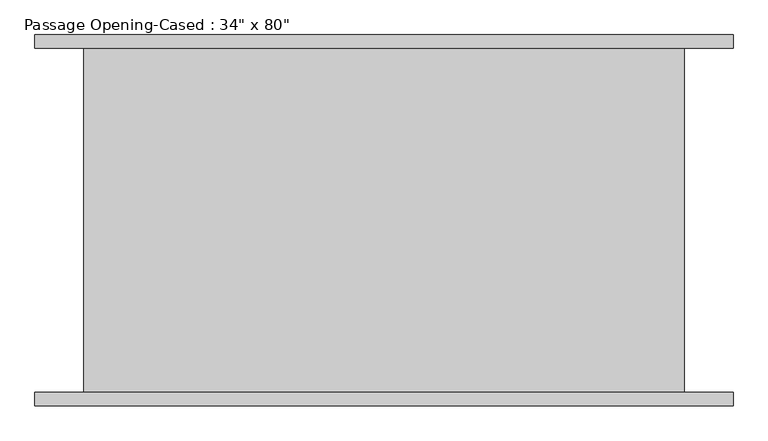
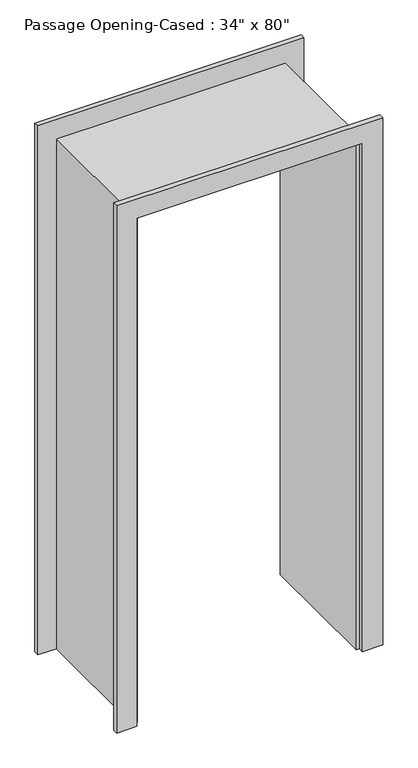
"""IFC4 building model written with IfcOpenShell, lengths in millimetres: proxy geometry."""

from ifc_helpers import new_model, si_unit, frame, origin, place, context, project, spatial, polyline, outline, extrude, faceted_brep, source, transform, mapped, element, save


def proxy_61b564c4(model_context):
    return source(origin(), model_context, "Body", "SolidModel", [
        extrude(outline(polyline([(0.0, -433.6386567), (2025.65, -433.6386567), (2025.65, 417.2613433), (0.0, 417.2613433), (0.0, 493.4613433), (2101.85, 493.4613433), (2101.85, -509.8386567), (0.0, -509.8386567), (0.0, -433.6386567)])), frame((0.0, -266.7, 0.0), z_axis=(0.0, 1.0, 0.0), x_axis=(0.0, 0.0, 1.0)), (0.0, 0.0, 1.0), 19.05),
        extrude(outline(polyline([(0.0, 493.4613433), (2108.2, 493.4613433), (2108.2, -509.8386567), (0.0, -509.8386567), (0.0, -433.6386567), (2025.65, -433.6386567), (2025.65, 417.2613433), (0.0, 417.2613433), (0.0, 493.4613433)])), frame((0.0, 247.65, 0.0), z_axis=(0.0, 1.0, 0.0), x_axis=(0.0, 0.0, 1.0)), (0.0, 0.0, 1.0), 19.05),
        faceted_brep([(404.5613433, 247.65, 0.0), (423.6113433, 247.65, 0.0), (423.6113433, -247.65, 0.0), (404.5613433, -247.65, 0.0), (404.5613433, 247.65, 2012.95), (423.6113433, 247.65, 2032.0), (423.6113433, -247.65, 2032.0), (404.5613433, -247.65, 2012.95), (-420.9386567, 247.65, 2012.95), (-439.9886567, 247.65, 2032.0), (-439.9886567, -247.65, 2032.0), (-420.9386567, -247.65, 2012.95), (-420.9386567, 247.65, 0.0), (-420.9386567, -247.65, 0.0), (-439.9886567, -247.65, 0.0), (-439.9886567, 247.65, 0.0)], [[[0, 1, 2, 3]], [[1, 0, 4, 5]], [[2, 1, 5, 6]], [[3, 2, 6, 7]], [[0, 3, 7, 4]], [[5, 4, 8, 9]], [[6, 5, 9, 10]], [[7, 6, 10, 11]], [[4, 7, 11, 8]], [[12, 13, 14, 15]], [[9, 8, 12, 15]], [[10, 9, 15, 14]], [[11, 10, 14, 13]], [[8, 11, 13, 12]]]),
    ])


if __name__ == "__main__":
    model = new_model("IFC4")
    model_context = context("Model", 3, world=origin())
    ifc_project = project(units=[si_unit("LENGTHUNIT", "METRE", prefix="MILLI")], contexts=[model_context])
    site = spatial("IfcSite", under=ifc_project)
    building = spatial("IfcBuilding", under=site)
    placement = place(None, origin())
    proxy_shape = proxy_61b564c4(model_context)
    element("IfcBuildingElementProxy", 1, Name="Passage Opening-Cased : 34\" x 80\"", ObjectType="Passage Opening-Cased : 34\" x 80\"", at=placement, inside=building, context=model_context, shape_type="MappedRepresentation", body=[
        mapped(proxy_shape, transform((0.0, 0.0, 0.0), x_axis=(1.0, 0.0, 0.0), y_axis=(0.0, 1.0, 0.0), z_axis=(0.0, 0.0, 1.0))),
    ])
    save(model, "model.ifc")

# Revit data of these elements
# Type "Passage Opening-Cased : 34\" x 80\""
#   Type Mark = "36"
#   Height = 6' - 8"
#   Trim Thickness = 0' - 0 3/4"
#   Trim Width = 0' - 3"
#   Width = 2' - 10"
#   Frame Material = Door - Frame
#   Default Elevation = 0
# Element 1 (IfcBuildingElementProxy, "Passage Opening-Cased : 34\" x 80\"")
#   Materials on its faces: "Door - Frame"
# Materials
#   "Door - Frame": class "Unassigned", colour RGB 118 70 51, transparency 0
